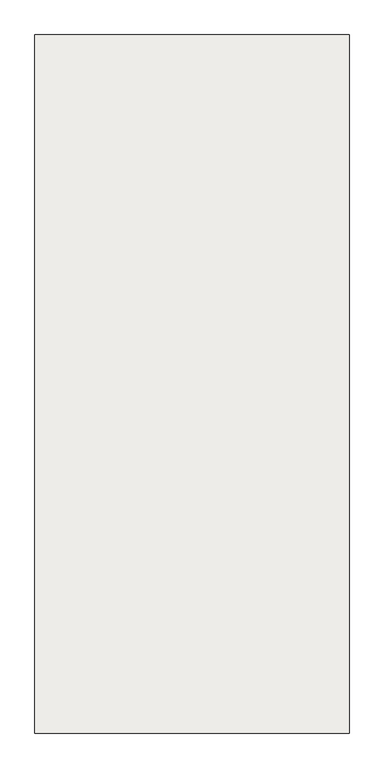
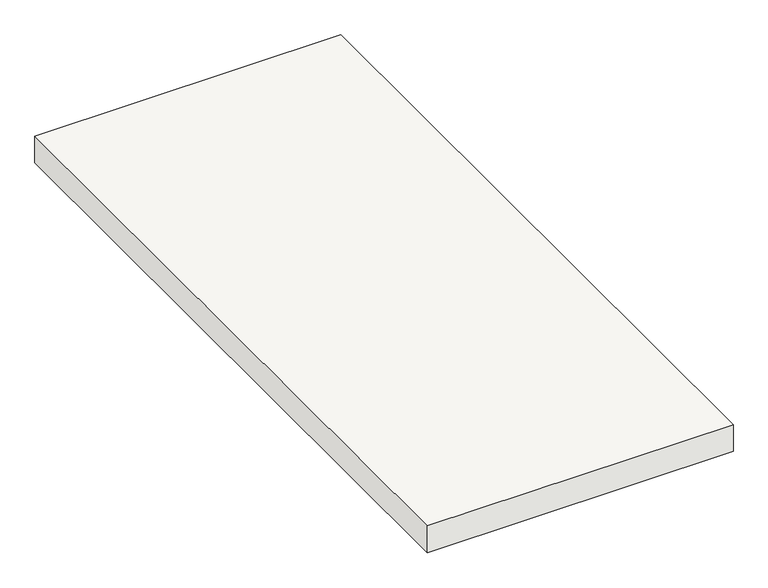
"""IFC4 building model written with IfcOpenShell, lengths in millimetres: slab geometry."""

from ifc_helpers import new_model, si_unit, frame, origin, place, context, project, spatial, polyline, outline, extrude, source, transform, mapped, element, save


def slab_19d7916a(model_context):
    return source(origin(), model_context, "Body", "SweptSolid", [
        extrude(outline(polyline([(6309.5374538, 37232.6086665), (6849.5374538, 37232.6086665), (6849.5374538, 36032.6086665), (6309.5374538, 36032.6086665), (6309.5374538, 37232.6086665)])), frame((0.0, 0.0, 4549.9720055), z_axis=(0.0, 0.0, 1.0), x_axis=(1.0, 0.0, 0.0)), (0.0, 0.0, 1.0), 50.0),
    ])


if __name__ == "__main__":
    model = new_model("IFC4")
    model_context = context("Model", 3, world=origin())
    ifc_project = project(units=[si_unit("LENGTHUNIT", "METRE", prefix="MILLI")], contexts=[model_context])
    site = spatial("IfcSite", under=ifc_project)
    building = spatial("IfcBuilding", under=site)
    placement = place(None, origin())
    slab_shape = slab_19d7916a(model_context)
    element("IfcSlab", 1, at=placement, inside=building, context=model_context, shape_type="MappedRepresentation", body=[
        mapped(slab_shape, transform((0.0, 0.0, 0.0), x_axis=(1.0, 0.0, 0.0), y_axis=(0.0, 1.0, 0.0), z_axis=(0.0, 0.0, 1.0))),
    ])
    save(model, "model.ifc")
